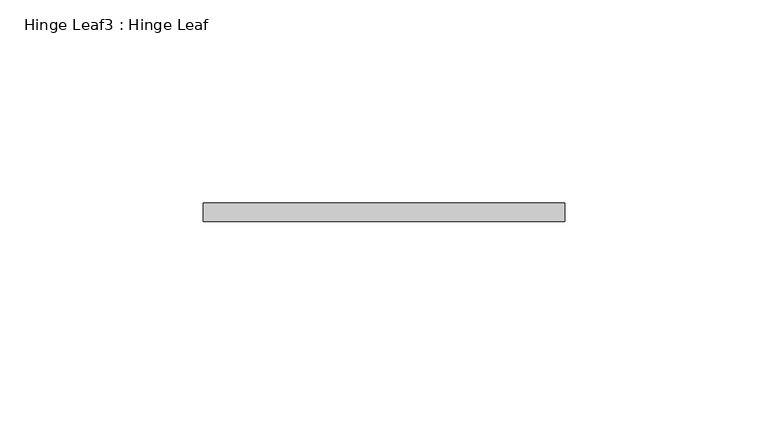
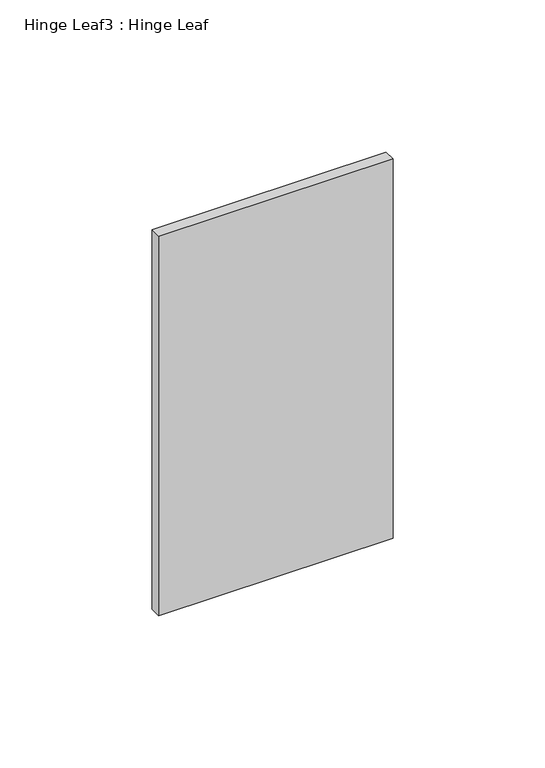
"""IFC4 building model written with IfcOpenShell, lengths in millimetres: proxy geometry, Hinge Leaf3 : Hinge Leaf."""

from ifc_helpers import new_model, si_unit, frame, origin, place, context, project, spatial, polyline, outline, extrude, source, transform, mapped, element, save


def hinge_leaf3_hinge_leaf_4683ff22(model_context):
    return source(origin(), model_context, "Body", "SweptSolid", [
        extrude(outline(polyline([(587327.7934739, -531772.5663841), (587416.6934739, -531772.5663841), (587416.6934739, -531777.1383841), (587327.7934739, -531777.1383841), (587327.7934739, -531772.5663841)])), frame((0.0, 0.0, 311.15), z_axis=(0.0, 0.0, 1.0), x_axis=(1.0, 0.0, 0.0)), (0.0, 0.0, 1.0), 152.4),
    ])


if __name__ == "__main__":
    model = new_model("IFC4")
    model_context = context("Model", 3, world=origin())
    ifc_project = project(units=[si_unit("LENGTHUNIT", "METRE", prefix="MILLI")], contexts=[model_context])
    site = spatial("IfcSite", under=ifc_project)
    building = spatial("IfcBuilding", under=site)
    placement = place(None, origin())
    hinge_leaf3_hinge_leaf_shape = hinge_leaf3_hinge_leaf_4683ff22(model_context)
    element("IfcBuildingElementProxy", 1, Name="Hinge Leaf3 : Hinge Leaf", ObjectType="Hinge Leaf3 : Hinge Leaf", at=placement, inside=building, context=model_context, shape_type="MappedRepresentation", body=[
        mapped(hinge_leaf3_hinge_leaf_shape, transform((0.0, 0.0, 0.0), x_axis=(1.0, 0.0, 0.0), y_axis=(0.0, 1.0, 0.0), z_axis=(0.0, 0.0, 1.0))),
    ])
    save(model, "model.ifc")

# Revit data of these elements
# Element 1 (IfcBuildingElementProxy, "Hinge Leaf3 : Hinge Leaf")
#   Materials on its faces: "6\"X6\" WELD-ON STL BUTT HINGE"
# Materials
#   "6\"X6\" WELD-ON STL BUTT HINGE": class "Metal", colour RGB 189 187 185, transparency 0, Description = "Carbon steel", Cost = 0
